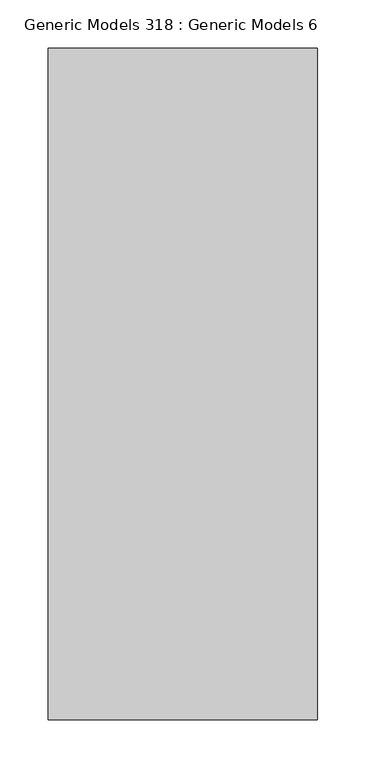
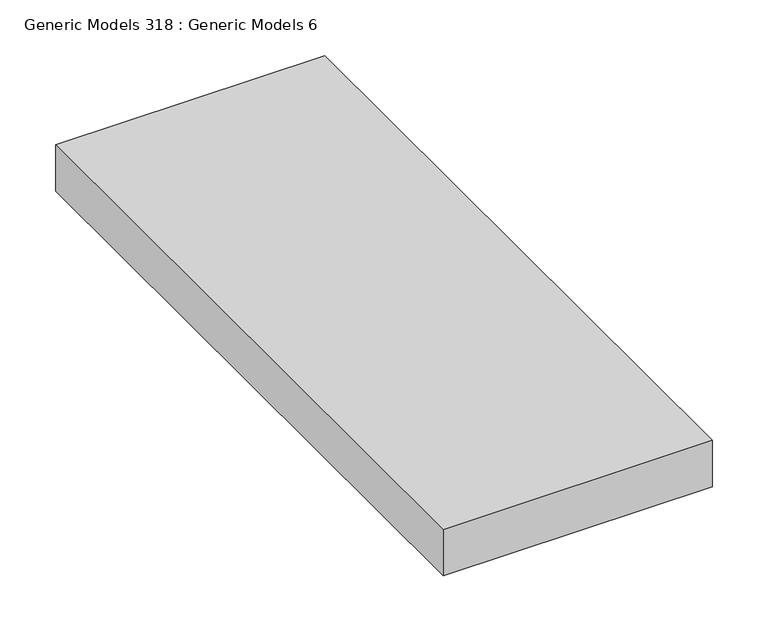
"""IFC4 building model written with IfcOpenShell, lengths in millimetres: proxy geometry, Generic Models 318 : Generic Models 6."""

from ifc_helpers import new_model, si_unit, frame, origin, place, context, project, spatial, polyline, outline, extrude, source, transform, mapped, element, save


def generic_models_318_generic_models_6_f48faca8(model_context):
    return source(origin(), model_context, "Body", "SweptSolid", [
        extrude(outline(polyline([(5397.3263704, 1095.7884092), (5676.7263704, 1095.7884092), (5676.7263704, 399.7309662), (5397.3263704, 399.7309662), (5397.3263704, 1095.7884092)])), frame((0.0, 0.0, 126599.696), z_axis=(0.0, 0.0, 1.0), x_axis=(1.0, 0.0, 0.0)), (0.0, 0.0, 1.0), 50.8),
    ])


if __name__ == "__main__":
    model = new_model("IFC4")
    model_context = context("Model", 3, world=origin())
    ifc_project = project(units=[si_unit("LENGTHUNIT", "METRE", prefix="MILLI")], contexts=[model_context])
    site = spatial("IfcSite", under=ifc_project)
    building = spatial("IfcBuilding", under=site)
    placement = place(None, origin())
    generic_models_318_generic_models_6_shape = generic_models_318_generic_models_6_f48faca8(model_context)
    element("IfcBuildingElementProxy", 1, Name="Generic Models 318 : Generic Models 6", ObjectType="Generic Models 318 : Generic Models 6", at=placement, inside=building, context=model_context, shape_type="MappedRepresentation", body=[
        mapped(generic_models_318_generic_models_6_shape, transform((0.0, 0.0, 0.0), x_axis=(1.0, 0.0, 0.0), y_axis=(0.0, 1.0, 0.0), z_axis=(0.0, 0.0, 1.0))),
    ])
    save(model, "model.ifc")

# Revit data of these elements
# Element 1 (IfcBuildingElementProxy, "Generic Models 318 : Generic Models 6")
#   Materials on its faces: "_HARDWOOD TREADS, SPECIES AND FINISH PER OWNER"
# Materials
#   "_HARDWOOD TREADS, SPECIES AND FINISH PER OWNER": class "Generic", colour RGB 177 130 114, transparency 0, Cost = 0
